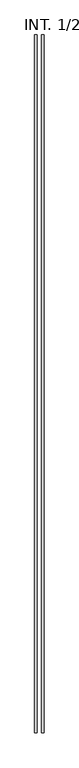
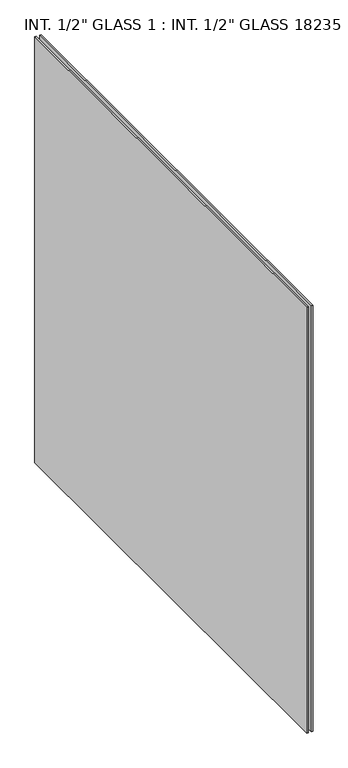
"""IFC4 building model written with IfcOpenShell, lengths in millimetres: proxy geometry."""

from ifc_helpers import new_model, si_unit, frame, origin, place, context, project, spatial, polyline, outline, extrude, source, transform, mapped, element, save


def proxy_6b060856(model_context):
    return source(origin(), model_context, "Body", "SweptSolid", [
        extrude(outline(polyline([(7615.184586, -1748.0991938), (7621.534586, -1748.0991938), (7621.534586, -3747.9491938), (7615.184586, -3747.9491938), (7615.184586, -1748.0991938)])), frame((0.0, 0.0, 37606.8963912), z_axis=(0.0, 0.0, 1.0), x_axis=(1.0, 0.0, 0.0)), (0.0, 0.0, 1.0), 1909.0140118),
        extrude(outline(polyline([(7595.0330695, -1748.0991938), (7601.3830695, -1748.0991938), (7601.3830695, -3747.9491938), (7595.0330695, -3747.9491938), (7595.0330695, -1748.0991938)])), frame((0.0, 0.0, 37606.8963912), z_axis=(0.0, 0.0, 1.0), x_axis=(1.0, 0.0, 0.0)), (0.0, 0.0, 1.0), 1909.0140118),
    ])


if __name__ == "__main__":
    model = new_model("IFC4")
    model_context = context("Model", 3, world=origin())
    ifc_project = project(units=[si_unit("LENGTHUNIT", "METRE", prefix="MILLI")], contexts=[model_context])
    site = spatial("IfcSite", under=ifc_project)
    building = spatial("IfcBuilding", under=site)
    placement = place(None, origin())
    proxy_shape = proxy_6b060856(model_context)
    element("IfcBuildingElementProxy", 1, Name="INT. 1/2\" GLASS 1 : INT. 1/2\" GLASS 18235", ObjectType="INT. 1/2\" GLASS 1 : INT. 1/2\" GLASS 18235", at=placement, inside=building, context=model_context, shape_type="MappedRepresentation", body=[
        mapped(proxy_shape, transform((0.0, 0.0, 0.0), x_axis=(1.0, 0.0, 0.0), y_axis=(0.0, 1.0, 0.0), z_axis=(0.0, 0.0, 1.0))),
    ])
    save(model, "model.ifc")

# Revit data of these elements
# Type "INT. 1/2\" GLASS 1 : INT. 1/2\" GLASS 18235"
#   NameOverride = "INT. 1/2\" GLASS"
# Element 1 (IfcBuildingElementProxy, "INT. 1/2\" GLASS 1 : INT. 1/2\" GLASS 18235")
#   Materials on its faces: "1/2\" TEMPERED GLASS"
# Materials
#   "1/2\" TEMPERED GLASS": class "Unassigned", colour RGB 191 240 251, transparency 0, Cost = 0
